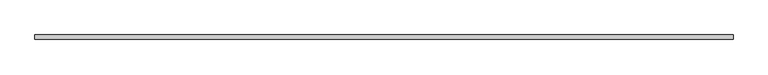
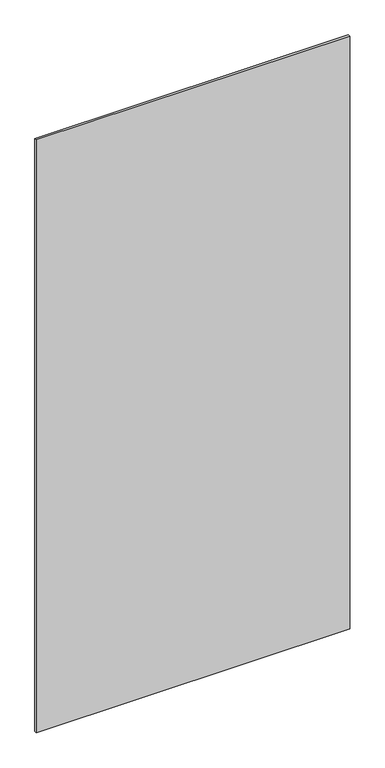
"""IFC4 building model written with IfcOpenShell, lengths in millimetres: proxy geometry, Panel:Panel:300402:Panel:300402 : Panel:Panel:300402:300124:Panel:300402:Panel:300402 : Panel:Panel:300402:300124 : Panel:Panel:300402:Panel:300402 : Panel:Panel:300402:300124:7 : Panel:Panel:300402:Panel:300402 : Panel:Panel:300402:300124:Panel:300402:Panel:300402 : Panel:Panel:300402:300124 : Panel:Panel:300402:Panel:300402 : Panel:Panel:300402:300124:300083."""

from ifc_helpers import new_model, si_unit, frame, origin, place, context, project, spatial, polyline, outline, extrude, source, transform, mapped, element, save


def generic_models_ccdbf5d9(model_context):
    return source(origin(), model_context, "Body", "SweptSolid", [
        extrude(outline(polyline([(569227.0867239, -579076.8913841), (570446.2867239, -579076.8913841), (570446.2867239, -579084.8288841), (569227.0867239, -579084.8288841), (569227.0867239, -579076.8913841)])), frame((0.0, 0.0, 3733.8), z_axis=(0.0, 0.0, 1.0), x_axis=(1.0, 0.0, 0.0)), (0.0, 0.0, 1.0), 2438.4),
    ])


if __name__ == "__main__":
    model = new_model("IFC4")
    model_context = context("Model", 3, world=origin())
    ifc_project = project(units=[si_unit("LENGTHUNIT", "METRE", prefix="MILLI")], contexts=[model_context])
    site = spatial("IfcSite", under=ifc_project)
    building = spatial("IfcBuilding", under=site)
    placement = place(None, origin())
    generic_models_shape = generic_models_ccdbf5d9(model_context)
    element("IfcBuildingElementProxy", 1, Name="Panel:Panel:300402:Panel:300402 : Panel:Panel:300402:300124:Panel:300402:Panel:300402 : Panel:Panel:300402:300124 : Panel:Panel:300402:Panel:300402 : Panel:Panel:300402:300124:7 : Panel:Panel:300402:Panel:300402 : Panel:Panel:300402:300124:Panel:300402:Panel:300402 : Panel:Panel:300402:300124 : Panel:Panel:300402:Panel:300402 : Panel:Panel:300402:300124:300083", ObjectType="Panel:Panel:300402:Panel:300402 : Panel:Panel:300402:300124:Panel:300402:Panel:300402 : Panel:Panel:300402:300124 : Panel:Panel:300402:Panel:300402 : Panel:Panel:300402:300124:7 : Panel:Panel:300402:Panel:300402 : Panel:Panel:300402:300124:Panel:300402:Panel:300402 : Panel:Panel:300402:300124 : Panel:Panel:300402:Panel:300402 : Panel:Panel:300402:300124:300083", at=placement, inside=building, context=model_context, shape_type="MappedRepresentation", body=[
        mapped(generic_models_shape, transform((0.0, 0.0, 0.0), x_axis=(1.0, 0.0, 0.0), y_axis=(0.0, 1.0, 0.0), z_axis=(0.0, 0.0, 1.0))),
    ])
    save(model, "model.ifc")

# Revit data of these elements
# Type "Panel:Panel:300402:Panel:300402 : Panel:Panel:300402:300124:Panel:300402:Panel:300402 : Panel:Panel:300402:300124 : Panel:Panel:300402:Panel:300402 : Panel:Panel:300402:300124:7 : Panel:Panel:300402:Panel:300402 : Panel:Panel:300402:300124:Panel:300402:Panel:300402 : Panel:Panel:300402:300124 : Panel:Panel:300402:Panel:300402 : Panel:Panel:300402:300124:300083"
#   NameOverride = "Panel:Panel:300402:Panel:300402 : Panel:Panel:300402:300124:Panel:300402:Panel:300402 : Panel:Panel:300402:300124 : Panel:Panel:300402:Panel:300402 : Panel:Panel:300402:300124:300083"
#   ObjectTypeOverride = "Panel:300402:Panel:300402 : Panel:Panel:300402:300124 : Panel:Panel:300402:Panel:300402 : Panel:Panel:300402:300124"
#   Reference = "Panel"
#   Tag = "300083"
# Element 1 (IfcBuildingElementProxy, "Panel:Panel:300402:Panel:300402 : Panel:Panel:300402:300124:Panel:300402:Panel:300402 : Panel:Panel:300402:300124 : Panel:Panel:300402:Panel:300402 : Panel:Panel:300402:300124:7 : Panel:Panel:300402:Panel:300402 : Panel:Panel:300402:300124:Panel:300402:Panel:300402 : Panel:Panel:300402:300124 : Panel:Panel:300402:Panel:300402 : Panel:Panel:300402:300124:300083")
#   Materials on its faces: "5/16\" THICK STONEWOOD RESIN PANELS - EXPOSED FASTENERS"
# Materials
#   "5/16\" THICK STONEWOOD RESIN PANELS - EXPOSED FASTENERS": class "Unassigned", colour RGB 64 64 64, transparency 0, Keynote = "M07420000.01", Cost = 0
